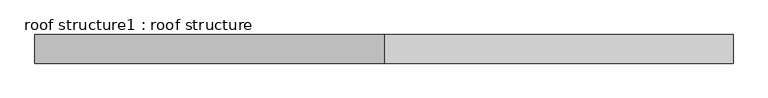
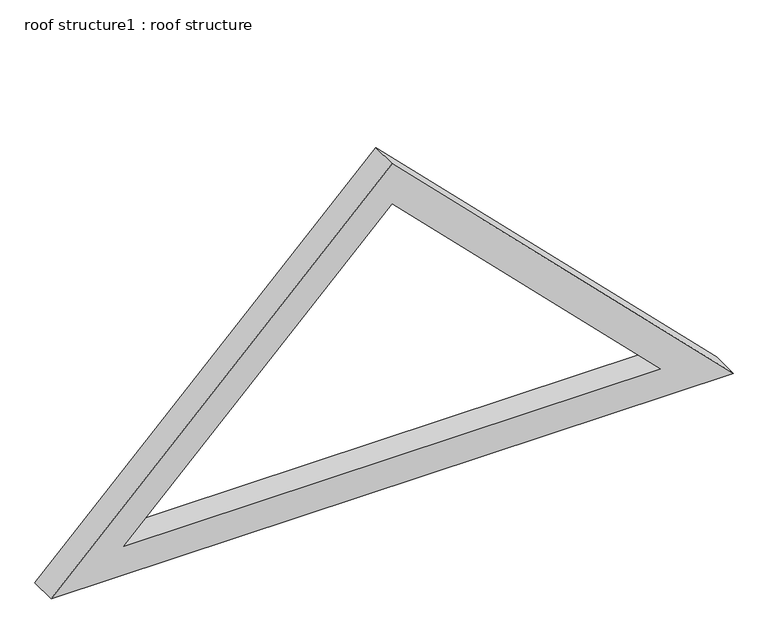
"""IFC4 building model written with IfcOpenShell, lengths in millimetres: beam geometry, roof structure1 : roof structure."""

from ifc_helpers import new_model, si_unit, frame, origin, place, context, project, spatial, polyline, outline, extrude, source, transform, mapped, element, save


def roof_structure1_roof_structure_631497e4(model_context):
    return source(origin(), model_context, "Body", "SweptSolid", [
        extrude(outline(polyline([(6191.25, 21451.0870052), (4471.162, 19730.9990052), (4471.162, 23171.1750052), (6191.25, 21451.0870052)]), holes=[polyline([(5975.7238531, 21451.0870052), (4623.562, 22803.2488583), (4623.562, 20098.9251521), (5975.7238531, 21451.0870052)])]), frame((0.0, 1323.8237428, 0.0), z_axis=(0.0, 1.0, 0.0), x_axis=(0.0, 0.0, 1.0)), (0.0, 0.0, 1.0), 140.99525),
    ])


if __name__ == "__main__":
    model = new_model("IFC4")
    model_context = context("Model", 3, world=origin())
    ifc_project = project(units=[si_unit("LENGTHUNIT", "METRE", prefix="MILLI")], contexts=[model_context])
    site = spatial("IfcSite", under=ifc_project)
    building = spatial("IfcBuilding", under=site)
    placement = place(None, origin())
    roof_structure1_roof_structure_shape = roof_structure1_roof_structure_631497e4(model_context)
    element("IfcBeam", 1, ObjectType="roof structure1 : roof structure", at=placement, inside=building, context=model_context, shape_type="MappedRepresentation", body=[
        mapped(roof_structure1_roof_structure_shape, transform((0.0, 0.0, 0.0), x_axis=(1.0, 0.0, 0.0), y_axis=(0.0, 1.0, 0.0), z_axis=(0.0, 0.0, 1.0))),
    ])
    save(model, "model.ifc")

# Revit data of these elements
# Element 1 (IfcBeam, "roof structure1 : roof structure")
#   Materials on its faces: "6X6 WOOD COLUMNS"
# Materials
#   "6X6 WOOD COLUMNS": class "Generic", colour RGB 227 170 128, transparency 0, Cost = 0
